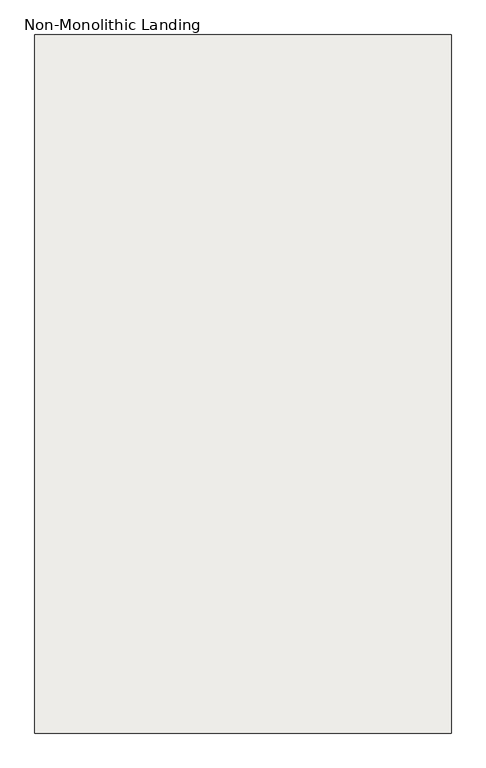
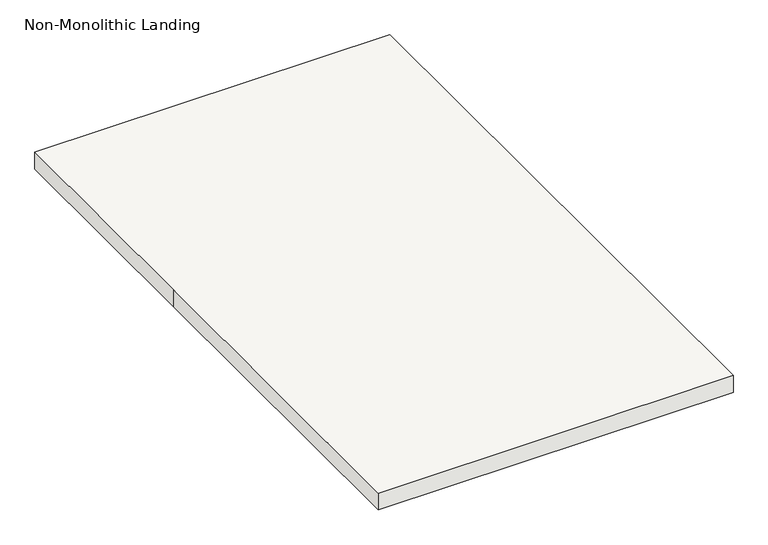
"""IFC4 building model written with IfcOpenShell, lengths in millimetres: slab geometry, Non-Monolithic Landing."""

from ifc_helpers import new_model, si_unit, frame, origin, place, context, project, spatial, polyline, outline, extrude, source, transform, mapped, element, save


def non_monolithic_landing_293fa1f8(model_context):
    return source(origin(), model_context, "Body", "SweptSolid", [
        extrude(outline(polyline([(21549.836337, -2576.2808257), (21549.836337, -1900.524372), (22549.836337, -1900.524372), (22549.836337, -3576.2808257), (21549.836337, -3576.2808257), (21549.836337, -2576.2808257)])), frame((0.0, 0.0, 1859.0909091), z_axis=(0.0, 0.0, 1.0), x_axis=(1.0, 0.0, 0.0)), (0.0, 0.0, 1.0), 50.0),
    ])


if __name__ == "__main__":
    model = new_model("IFC4")
    model_context = context("Model", 3, world=origin())
    ifc_project = project(units=[si_unit("LENGTHUNIT", "METRE", prefix="MILLI")], contexts=[model_context])
    site = spatial("IfcSite", under=ifc_project)
    building = spatial("IfcBuilding", under=site)
    placement = place(None, origin())
    non_monolithic_landing_shape = non_monolithic_landing_293fa1f8(model_context)
    element("IfcSlab", 1, ObjectType="Non-Monolithic Landing", at=placement, inside=building, context=model_context, shape_type="MappedRepresentation", body=[
        mapped(non_monolithic_landing_shape, transform((0.0, 0.0, 0.0), x_axis=(1.0, 0.0, 0.0), y_axis=(0.0, 1.0, 0.0), z_axis=(0.0, 0.0, 1.0))),
    ])
    save(model, "model.ifc")
